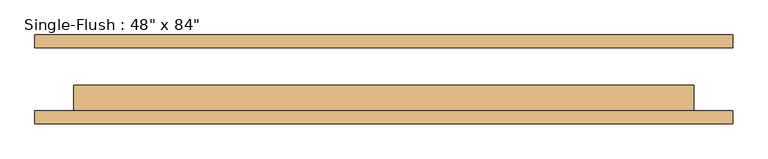
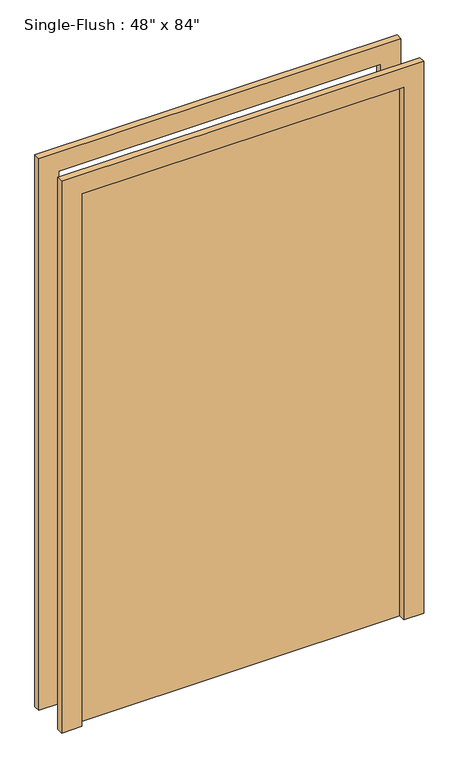
"""IFC4 building model written with IfcOpenShell, lengths in millimetres: door geometry."""

from ifc_helpers import new_model, si_unit, frame, origin, origin_with_axes, place, context, project, spatial, polyline, outline, extrude, source, transform, mapped, element, save


def door_1f4748c7(model_context):
    return source(origin(), model_context, "Body", "SweptSolid", [
        extrude(outline(polyline([(2209.8, -685.8), (0.0, -685.8), (0.0, -609.6), (2133.6, -609.6), (2133.6, 609.6), (0.0, 609.6), (0.0, 685.8), (2209.8, 685.8), (2209.8, -685.8)])), frame((0.0, -87.3125, 0.0), z_axis=(0.0, 1.0, 0.0), x_axis=(0.0, 0.0, 1.0)), (0.0, 0.0, 1.0), 25.4),
        extrude(outline(polyline([(2209.8, 685.8), (2209.8, -685.8), (0.0, -685.8), (0.0, -609.6), (2133.6, -609.6), (2133.6, 609.6), (0.0, 609.6), (0.0, 685.8), (2209.8, 685.8)])), frame((0.0, 61.9125, 0.0), z_axis=(0.0, 1.0, 0.0), x_axis=(0.0, 0.0, 1.0)), (0.0, 0.0, 1.0), 25.4),
        extrude(outline(polyline([(609.6, -11.1125), (609.6, -61.9125), (-609.6, -61.9125), (-609.6, -11.1125), (609.6, -11.1125)])), origin_with_axes(), (0.0, 0.0, 1.0), 2133.6),
    ])


if __name__ == "__main__":
    model = new_model("IFC4")
    model_context = context("Model", 3, world=origin())
    ifc_project = project(units=[si_unit("LENGTHUNIT", "METRE", prefix="MILLI")], contexts=[model_context])
    site = spatial("IfcSite", under=ifc_project)
    building = spatial("IfcBuilding", under=site)
    placement = place(None, origin())
    door_shape = door_1f4748c7(model_context)
    element("IfcDoor", 1, ObjectType="Single-Flush : 48\" x 84\"", at=placement, inside=building, context=model_context, shape_type="MappedRepresentation", body=[
        mapped(door_shape, transform((0.0, 0.0, 0.0), x_axis=(1.0, 0.0, 0.0), y_axis=(0.0, 1.0, 0.0), z_axis=(0.0, 0.0, 1.0))),
    ])
    save(model, "model.ifc")

# Revit data of these elements
# Type "Single-Flush : 48\" x 84\""
#   Type Mark = "8"
#   Construction Type = "C"
#   Assembly Code = "C1020"
#   Thickness = 0' - 2"
#   Height = 7' - 0"
#   Trim Projection Ext = 0' - 1"
#   Trim Projection Int = 0' - 1"
#   Trim Width = 0' - 3"
#   Width = 4' - 0"
#   Door Material = Door - Panel
#   Frame Material = Door - Frame
#   Function = (empty or 0)
#   Wall Closure = (empty or 0)
# Element 1 (IfcDoor, "Single-Flush : 48\" x 84\"")
#   Materials on its faces: "Door - Frame", "Door - Panel"
# Materials
#   "Door - Panel": class "Wood", colour RGB 210 159 95, transparency 0
#   "Door - Frame": class "Miscellaneous", colour RGB 118 70 51, transparency 0
